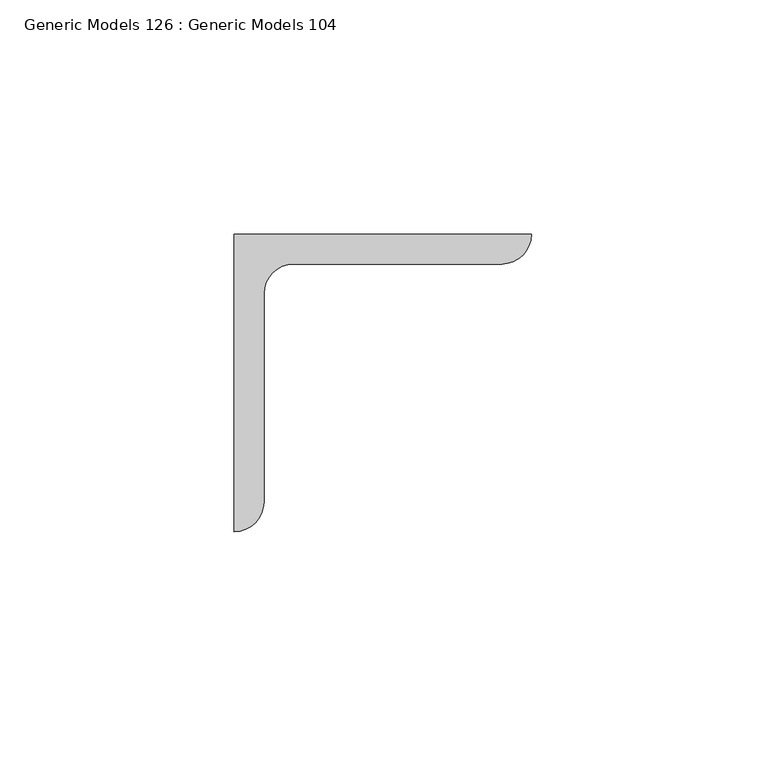
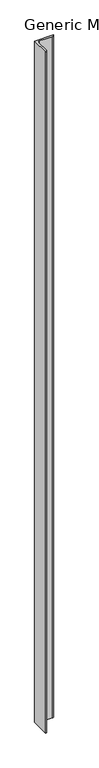
"""IFC4 building model written with IfcOpenShell, lengths in millimetres: proxy geometry, Generic Models 126 : Generic Models 104."""

import ifcopenshell
import ifcopenshell.guid

model = None  # the IFC model being written
_history = None  # IfcOwnerHistory: only IFC2X3 demands one
_inside = {}  # id of a spatial element -> (the spatial element, [elements in it])
_under = {}  # id of a project, library or spatial element -> (it, [spatial elements below it])
_declared = {}  # id of a project -> (the project, [libraries it declares])
_typed = {}  # id of a type object -> (the type object, [elements of that type])
_made_of = {}  # id of a material, layer set ... -> (it, [elements and type objects made of it])


def new_model(schema):
    """Start an empty IFC model of exactly this schema.

    Asked for "IFC4X3", IfcOpenShell would pick the latest addendum, in which some entities
    have other attributes; the version numbers below select the first issue.
    IFC2X3 requires an IfcOwnerHistory on every rooted entity: one is made here for all.
    """
    global model, _history
    if schema == "IFC4X3":
        model = ifcopenshell.file(schema_version=(4, 3, 0, 0))
    else:
        model = ifcopenshell.file(schema=schema)
    _inside.clear()
    _under.clear()
    _declared.clear()
    _typed.clear()
    _made_of.clear()
    _history = None
    if model.schema == "IFC2X3":
        org = make("IfcOrganization", Name="unknown")
        user = make(
            "IfcPersonAndOrganization",
            ThePerson=make("IfcPerson", FamilyName="unknown"),
            TheOrganization=org,
        )
        app = make(
            "IfcApplication",
            ApplicationDeveloper=org,
            Version="unknown",
            ApplicationFullName="unknown",
            ApplicationIdentifier="unknown",
        )
        _history = make(
            "IfcOwnerHistory",
            OwningUser=user,
            OwningApplication=app,
            ChangeAction="ADDED",
            CreationDate=0,
        )
    return model


def make(cls, **values):
    """One entity of the class cls with the attributes given. An attribute that is None is left unset."""
    return model.create_entity(
        cls, **{name: value for name, value in values.items() if value is not None}
    )


def rooted(cls, **values):
    """An entity with a GlobalId (a new one), such as an element, a storey or a relation."""
    return make(cls, GlobalId=ifcopenshell.guid.new(), OwnerHistory=_history, **values)


def si_unit(unit_type, name, prefix=None):
    """IfcSIUnit, for example si_unit("LENGTHUNIT", "METRE", prefix="MILLI")."""
    return make("IfcSIUnit", UnitType=unit_type, Prefix=prefix, Name=name)


def assignment(units):
    """IfcUnitAssignment: the units of a project."""
    return None if units is None else make("IfcUnitAssignment", Units=units)


def point(xyz):
    """IfcCartesianPoint."""
    return None if xyz is None else make("IfcCartesianPoint", Coordinates=xyz)


def direction(xyz):
    """IfcDirection."""
    return None if xyz is None else make("IfcDirection", DirectionRatios=xyz)


def frame(location, z_axis=None, x_axis=None):
    """IfcAxis2Placement3D, a coordinate frame: its origin and axes. An axis left out is left unset."""
    return make(
        "IfcAxis2Placement3D",
        Location=point(location),
        Axis=direction(z_axis),
        RefDirection=direction(x_axis),
    )


def frame_2d(location, x_axis=None):
    """IfcAxis2Placement2D, a coordinate frame in the plane: its origin and x axis."""
    return make(
        "IfcAxis2Placement2D", Location=point(location), RefDirection=direction(x_axis)
    )


def origin():
    """The frame at (0, 0, 0) with its axes left unset."""
    return frame((0.0, 0.0, 0.0))


def place(relative_to, where):
    """IfcLocalPlacement: puts the frame where relative to a parent placement (None: the world)."""
    return make(
        "IfcLocalPlacement", PlacementRelTo=relative_to, RelativePlacement=where
    )


def context(
    kind, dimensions, precision=None, world=None, true_north=None, identifier=None
):
    """IfcGeometricRepresentationContext, for example the 3D "Model" context."""
    return make(
        "IfcGeometricRepresentationContext",
        ContextIdentifier=identifier,
        ContextType=kind,
        CoordinateSpaceDimension=dimensions,
        Precision=precision,
        WorldCoordinateSystem=world,
        TrueNorth=true_north,
    )


def project(units=None, contexts=None):
    """IfcProject with its units and contexts."""
    return rooted(
        "IfcProject",
        Name="project",
        RepresentationContexts=contexts,
        UnitsInContext=assignment(units),
    )


def spatial(cls, under=None, at=None, **own):
    """A site, building, storey or space (cls), placed at a placement, below another one or the project."""
    s = rooted(cls, ObjectPlacement=at, **own)
    if under is not None:
        _under.setdefault(under.id(), (under, []))[1].append(s)
    return s


def polyline(points):
    """IfcPolyline through the points."""
    return make("IfcPolyline", Points=[point(p) for p in points])


def circle_curve(where, radius):
    """IfcCircle in the frame where."""
    return make("IfcCircle", Position=where, Radius=radius)


def trimmed(basis, trim1, trim2, sense, master):
    """IfcTrimmedCurve: the piece of a basis curve between two trims."""
    return make(
        "IfcTrimmedCurve",
        BasisCurve=basis,
        Trim1=trim1,
        Trim2=trim2,
        SenseAgreement=sense,
        MasterRepresentation=master,
    )


def segment(curve, same_sense, transition):
    """IfcCompositeCurveSegment."""
    return make(
        "IfcCompositeCurveSegment",
        Transition=transition,
        SameSense=same_sense,
        ParentCurve=curve,
    )


def composite_curve(segments, self_intersect=None):
    """IfcCompositeCurve: segments joined end to end."""
    return make("IfcCompositeCurve", Segments=segments, SelfIntersect=self_intersect)


def outline(outer, holes=None, kind="AREA"):
    """IfcArbitraryClosedProfileDef: a profile drawn as a closed curve; with holes, ...WithVoids."""
    if holes is None:
        return make("IfcArbitraryClosedProfileDef", ProfileType=kind, OuterCurve=outer)
    return make(
        "IfcArbitraryProfileDefWithVoids",
        ProfileType=kind,
        OuterCurve=outer,
        InnerCurves=holes,
    )


def extrude(swept, where, along, depth):
    """IfcExtrudedAreaSolid: the profile swept, set in the frame where, extruded along a direction by depth."""
    return make(
        "IfcExtrudedAreaSolid",
        SweptArea=swept,
        Position=where,
        ExtrudedDirection=direction(along),
        Depth=depth,
    )


def shape(context_of_items, identifier, shape_type, items):
    """IfcShapeRepresentation: the items that make up one representation, for example the "Body"."""
    return make(
        "IfcShapeRepresentation",
        ContextOfItems=context_of_items,
        RepresentationIdentifier=identifier,
        RepresentationType=shape_type,
        Items=items,
    )


def source(mapping_origin, context_of_items, identifier, shape_type, items):
    """IfcRepresentationMap: a shape defined once, which mapped items show again and again."""
    return make(
        "IfcRepresentationMap",
        MappingOrigin=mapping_origin,
        MappedRepresentation=shape(context_of_items, identifier, shape_type, items),
    )


def transform(
    local_origin,
    x_axis=None,
    y_axis=None,
    z_axis=None,
    scale=None,
    scale2=None,
    scale3=None,
    uniform=True,
):
    """IfcCartesianTransformationOperator3D, or its non-uniform kind. x_axis, y_axis, z_axis: its Axis1, 2, 3."""
    if uniform:
        return make(
            "IfcCartesianTransformationOperator3D",
            Axis1=direction(x_axis),
            Axis2=direction(y_axis),
            LocalOrigin=point(local_origin),
            Scale=scale,
            Axis3=direction(z_axis),
        )
    return make(
        "IfcCartesianTransformationOperator3DnonUniform",
        Axis1=direction(x_axis),
        Axis2=direction(y_axis),
        LocalOrigin=point(local_origin),
        Scale=scale,
        Axis3=direction(z_axis),
        Scale2=scale2,
        Scale3=scale3,
    )


def mapped(mapping_source, mapping_target):
    """IfcMappedItem: shows the shape of a source again, moved by a transform."""
    return make(
        "IfcMappedItem", MappingSource=mapping_source, MappingTarget=mapping_target
    )


def made_of(thing, what):
    """Note that an element or type object is made of a material, layer set ...; save() writes the relation."""
    if what is not None:
        _made_of.setdefault(what.id(), (what, []))[1].append(thing)
    return thing


def element(
    cls,
    number,
    at=None,
    inside=None,
    cuts=None,
    type_object=None,
    material=None,
    context=None,
    identifier="Body",
    shape_type=None,
    held_by="IfcProductDefinitionShape",
    body=None,
    shapes=None,
    **own,
):
    """One element of the class cls, such as IfcWall. Its Tag is "e" and its number.

    at: its placement. inside: the storey or other place that contains it. cuts: it is an
    opening in that element (IfcRelVoidsElement). A single representation is given by context,
    identifier, shape_type and body (its items); several are given by shapes. held_by: the class
    of the entity that holds the representations. save() writes the other relations.
    """
    e = rooted(cls, Tag="e%d" % number, ObjectPlacement=at, **own)
    if body is not None:
        shapes = [shape(context, identifier, shape_type, body)]
    if shapes is not None:
        e.Representation = make(held_by, Representations=shapes)
    if inside is not None:
        _inside.setdefault(inside.id(), (inside, []))[1].append(e)
    if cuts is not None:
        rooted(
            "IfcRelVoidsElement", RelatingBuildingElement=cuts, RelatedOpeningElement=e
        )
    if type_object is not None:
        _typed.setdefault(type_object.id(), (type_object, []))[1].append(e)
    return made_of(e, material)


def aggregate(whole, parts):
    """IfcRelAggregates: a whole, such as a stair, and the parts it consists of."""
    return rooted("IfcRelAggregates", RelatingObject=whole, RelatedObjects=parts)


def save(model, path):
    """Write the relations noted so far, then the file.

    IfcRelAggregates (storeys below a building ...), IfcRelContainedInSpatialStructure (elements
    in a storey), IfcRelDefinesByType, IfcRelAssociatesMaterial and IfcRelDeclares: one each for
    every whole, place, type object, material and project.
    """
    for whole, parts in _under.values():
        aggregate(whole, parts)
    for where, things in _inside.values():
        rooted(
            "IfcRelContainedInSpatialStructure",
            RelatedElements=things,
            RelatingStructure=where,
        )
    for kind, things in _typed.values():
        rooted("IfcRelDefinesByType", RelatedObjects=things, RelatingType=kind)
    for what, things in _made_of.values():
        rooted("IfcRelAssociatesMaterial", RelatedObjects=things, RelatingMaterial=what)
    for by, libraries in _declared.values():
        rooted("IfcRelDeclares", RelatingContext=by, RelatedDefinitions=libraries)
    model.write(path)


def generic_models_126_generic_models_104_9d8c6328(model_context):
    return source(origin(), model_context, "Body", "SweptSolid", [
        extrude(outline(composite_curve([segment(polyline([(28125.7340778, 41071.1196612), (28189.2340778, 41071.1196612)]), True, "CONTINUOUS"), segment(trimmed(circle_curve(frame_2d((28182.8840778, 41071.1196612)), 6.35), [point((28189.2340778, 41071.1196612))], [point((28182.8840778, 41064.7696612))], False, "CARTESIAN"), True, "CONTINUOUS"), segment(polyline([(28182.8840778, 41064.7696612), (28138.4340778, 41064.7696612)]), True, "CONTINUOUS"), segment(trimmed(circle_curve(frame_2d((28138.4340778, 41058.4196612)), 6.35), [point((28138.4340778, 41064.7696612))], [point((28132.0840778, 41058.4196612))], True, "CARTESIAN"), True, "CONTINUOUS"), segment(polyline([(28132.0840778, 41058.4196612), (28132.0840778, 41013.9696612)]), True, "CONTINUOUS"), segment(trimmed(circle_curve(frame_2d((28125.7340778, 41013.9696612)), 6.35), [point((28132.0840778, 41013.9696612))], [point((28125.7340778, 41007.6196612))], False, "CARTESIAN"), True, "CONTINUOUS"), segment(polyline([(28125.7340778, 41007.6196612), (28125.7340778, 41071.1196612)]), True, "CONTINUOUS")], self_intersect=False)), frame((0.0, 0.0, 266407.9), z_axis=(0.0, 0.0, 1.0), x_axis=(1.0, 0.0, 0.0)), (0.0, 0.0, 1.0), 2432.1044757),
    ])


if __name__ == "__main__":
    model = new_model("IFC4")
    model_context = context("Model", 3, world=origin())
    ifc_project = project(units=[si_unit("LENGTHUNIT", "METRE", prefix="MILLI")], contexts=[model_context])
    site = spatial("IfcSite", under=ifc_project)
    building = spatial("IfcBuilding", under=site)
    placement = place(None, origin())
    generic_models_126_generic_models_104_shape = generic_models_126_generic_models_104_9d8c6328(model_context)
    element("IfcBuildingElementProxy", 1, Name="Generic Models 126 : Generic Models 104", ObjectType="Generic Models 126 : Generic Models 104", at=placement, inside=building, context=model_context, shape_type="MappedRepresentation", body=[
        mapped(generic_models_126_generic_models_104_shape, transform((0.0, 0.0, 0.0), x_axis=(1.0, 0.0, 0.0), y_axis=(0.0, 1.0, 0.0), z_axis=(0.0, 0.0, 1.0))),
    ])
    save(model, "model.ifc")

# Revit data of these elements
# Element 1 (IfcBuildingElementProxy, "Generic Models 126 : Generic Models 104")
#   Materials on its faces: "(2) BACK/BACK GALVANIZED ANGLES (2) L2 1/2 X 2 1/2 X 1/4\")"
# Materials
#   "(2) BACK/BACK GALVANIZED ANGLES (2) L2 1/2 X 2 1/2 X 1/4\")": class "Unassigned", colour RGB 211 211 211, transparency 0, Cost = 0
